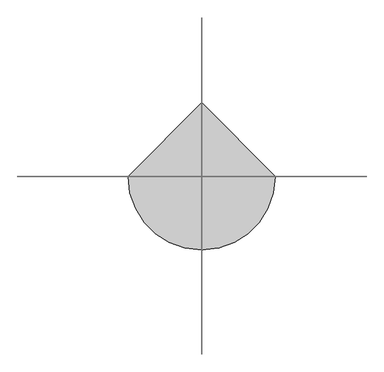
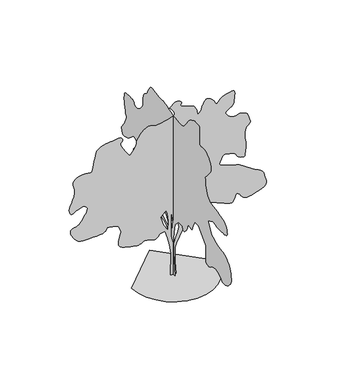
"""IFC4 building model written with IfcOpenShell, lengths in millimetres: geographic element geometry, RPC 木 - 落葉樹 : ブルーベリー エルダー - 4.5 メートル."""

from ifc_helpers import new_model, si_unit, origin, place, context, project, spatial, triangles, source, transform, mapped, element, save


def geographic_element_08da9c25(model_context):
    return source(origin(), model_context, "Body", "Tessellation", [
        triangles([(-0.0014684, 58.7037978, 0.0041346), (-0.0014684, -62.498052, 0.0041346), (-0.0014684, -15.3641626, 565.6129683), (-0.0014684, -1.8971866, 909.0182064), (-0.0014684, -22.0974929, 1104.2884094), (-0.0014684, -75.9650625, 1326.4911255), (-0.0014684, -224.1009287, 1474.6287403), (-0.0014684, -378.970291, 1474.6287403), (-0.0014684, -412.6378218, 1380.3586224), (-0.0014684, -479.9703761, 1387.0936764), (-0.0014684, -554.0404552, 1474.6287403), (-0.0014684, -601.1729708, 1568.8962421), (-0.0014684, -628.1080273, 1663.1638893), (-0.0014684, -702.1755266, 1636.2313763), (-0.0014684, -782.9756092, 1629.4963223), (-0.0014684, -857.0431812, 1797.8338669), (-0.0014684, -910.9107508, 1898.833952), (-0.0014684, -1059.0483656, 1892.1015141), (-0.0014684, -1173.5159426, 1797.8338669), (-0.0014684, -1382.2535648, 1575.6288254), (-0.0014684, -1388.9861481, 1353.4261093), (-0.0014684, -1386.9236286, 1327.021035), (-0.0014684, -1382.3910564, 1295.553479), (-0.0014684, -1377.8561588, 1261.3760593), (-0.0014684, -1375.7936394, 1226.8434288), (-0.0014684, -1378.6786377, 1194.3159811), (-0.0014684, -1388.9861481, 1166.1458982), (-0.0014684, -1409.1860779, 1144.6884144), (-0.0014684, -1434.4711624, 1129.1809307), (-0.0014684, -1458.931152, 1117.9109064), (-0.0014684, -1483.3911415, 1111.8258854), (-0.0014684, -1508.676226, 1111.8658539), (-0.0014684, -1535.6112099, 1118.9734142), (-0.0014684, -1565.0162464, 1134.0884073), (-0.0014684, -1597.723843, 1158.1559063), (-0.0014684, -1638.2812511, 1183.6959171), (-0.0014684, -1688.0263252, 1202.5209309), (-0.0014684, -1742.9539318, 1214.5159836), (-0.0014684, -1799.0589375, 1219.5610245), (-0.0014684, -1852.3364994, 1217.5409443), (-0.0014684, -1898.783955, 1208.3334394), (-0.0014684, -1934.3939907, 1191.8234734), (-0.0014684, -1963.8416119, 1167.0484594), (-0.0014684, -1995.1715309, 1136.2684341), (-0.0014684, -2029.446619, 1104.1908863), (-0.0014684, -2067.729166, 1075.5283916), (-0.0014684, -2111.0741947, 1054.9958513), (-0.0014684, -2160.5442856, 1047.2983561), (-0.0014684, -2217.1992577, 1057.1533504), (-0.0014684, -2275.1493542, 1083.4008762), (-0.0014684, -2327.094294, 1119.5408941), (-0.0014684, -2371.9694618, 1162.2784018), (-0.0014684, -2408.7193989, 1208.3134552), (-0.0014684, -2436.2819607, 1254.348436), (-0.0014684, -2453.5944214, 1297.0834728), (-0.0014684, -2459.6019035, 1333.2260342), (-0.0014684, -2455.754464, 1372.7236233), (-0.0014684, -2445.3120781, 1424.1161259), (-0.0014684, -2429.919413, 1481.9887562), (-0.0014684, -2411.2318909, 1540.9212055), (-0.0014684, -2390.8944695, 1595.4962173), (-0.0014684, -2370.5569027, 1640.2937737), (-0.0014684, -2351.8669098, 1669.8963272), (-0.0014684, -2330.1568977, 1694.4363991), (-0.0014684, -2300.1992786, 1725.2163517), (-0.0014684, -2262.8217636, 1758.5913494), (-0.0014684, -2218.8493023, 1790.903912), (-0.0014684, -2169.1042282, 1818.5039715), (-0.0014684, -2114.4116364, 1837.74146), (-0.0014684, -2055.5966217, 1844.9664551), (-0.0014684, -1994.4066067, 1849.8740044), (-0.0014684, -1932.1564819, 1863.6164795), (-0.0014684, -1869.0239983, 1884.7189705), (-0.0014684, -1805.1839996, 1911.7115089), (-0.0014684, -1740.8139462, 1943.1215103), (-0.0014684, -1676.0888271, 1977.4765354), (-0.0014684, -1611.1887188, 2013.3016743), (-0.0014684, -1469.786158, 2275.9068661), (-0.0014684, -1685.2562908, 2376.9094219), (-0.0014684, -1714.2713802, 2368.3093655), (-0.0014684, -1744.228854, 2360.0643745), (-0.0014684, -1776.0713871, 2352.5268986), (-0.0014684, -1810.7388931, 2346.049387), (-0.0014684, -1849.1765179, 2340.9844345), (-0.0014684, -1892.3265003, 2337.686816), (-0.0014684, -1941.1290447, 2336.5068008), (-0.0014684, -1996.881601, 2336.291843), (-0.0014684, -2057.3441895, 2336.4293346), (-0.0014684, -2118.1616982, 2338.0968201), (-0.0014684, -2174.9742188, 2342.4769306), (-0.0014684, -2223.421843, 2350.7393623), (-0.0014684, -2259.1517841, 2364.0693626), (-0.0014684, -2277.7993378, 2383.6418598), (-0.0014684, -2281.3742649, 2414.4819832), (-0.0014684, -2275.8767807, 2457.2194908), (-0.0014684, -2262.9592552, 2506.4269524), (-0.0014684, -2244.2692623, 2556.7020813), (-0.0014684, -2221.4593174, 2602.6271851), (-0.0014684, -2196.1742329, 2638.7770134), (-0.0014684, -2170.0641987, 2659.7021896), (-0.0014684, -2143.7191498, 2670.2021301), (-0.0014684, -2115.1367374, 2679.2771576), (-0.0014684, -2082.0791622, 2687.9772079), (-0.0014684, -2042.3065899, 2697.4022141), (-0.0014684, -1993.581657, 2708.6021118), (-0.0014684, -1933.6665642, 2722.6021294), (-0.0014684, -1860.3264187, 2740.5021996), (-0.0014684, -1781.7239491, 2758.3022758), (-0.0014684, -1708.0688519, 2773.1522415), (-0.0014684, -1640.1837513, 2787.8522163), (-0.0014684, -1578.8962132, 2805.302314), (-0.0014684, -1525.0287163, 2828.2773651), (-0.0014684, -1479.4062103, 2859.6021973), (-0.0014684, -1442.8536449, 2902.1272179), (-0.0014684, -1414.8411106, 2953.5272781), (-0.0014684, -1393.5411026, 3009.1773697), (-0.0014684, -1377.8361019, 3068.3775352), (-0.0014684, -1366.6061188, 3130.3775299), (-0.0014684, -1358.7336342, 3194.527684), (-0.0014684, -1353.1011292, 3260.0777527), (-0.0014684, -1348.5861431, 3326.3277786), (-0.0014684, -1398.7811897, 3378.2528069), (-0.0014684, -1447.1536732, 3430.0528427), (-0.0014684, -1491.8711472, 3481.6278923), (-0.0014684, -1531.1136646, 3532.8529633), (-0.0014684, -1563.0537209, 3583.577774), (-0.0014684, -1585.8662819, 3633.7529091), (-0.0014684, -1597.723843, 3683.2030884), (-0.0014684, -1593.7187096, 3737.8779488), (-0.0014684, -1572.2812099, 3799.8529449), (-0.0014684, -1536.5912373, 3863.2281464), (-0.0014684, -1489.8311554, 3922.153038), (-0.0014684, -1435.1786774, 3970.7032722), (-0.0014684, -1375.8135509, 4002.9783371), (-0.0014684, -1314.918576, 4013.128299), (-0.0014684, -1258.4585049, 4010.1031929), (-0.0014684, -1210.3634754, 4007.7533363), (-0.0014684, -1170.7484516, 4007.6533424), (-0.0014684, -1139.7309408, 4011.3281181), (-0.0014684, -1117.4309212, 4020.3031517), (-0.0014684, -1103.9633566, 4036.1033501), (-0.0014684, -1099.4483706, 4060.2783279), (-0.0014684, -1101.1558971, 4105.3531929), (-0.0014684, -1104.8659178, 4175.1532928), (-0.0014684, -1108.4583584, 4258.1534592), (-0.0014684, -1109.8133629, 4342.8035248), (-0.0014684, -1106.8083864, 4417.5536133), (-0.0014684, -1097.3283691, 4470.8785561), (-0.0014684, -1079.2483681, 4491.2034782), (-0.0014684, -1052.7858118, 4492.578685), (-0.0014684, -1020.9033102, 4495.6035004), (-0.0014684, -985.6082989, 4498.6286064), (-0.0014684, -948.8982576, 4500.0035225), (-0.0014684, -912.7757532, 4498.07864), (-0.0014684, -879.2456778, 4491.2034782), (-0.0014684, -850.3106707, 4477.7537178), (-0.0014684, -822.8281912, 4461.7535316), (-0.0014684, -792.8706448, 4447.2035477), (-0.0014684, -761.2631264, 4432.1535942), (-0.0014684, -728.8330564, 4414.7534935), (-0.0014684, -696.4030592, 4393.1286507), (-0.0014684, -664.7980116, 4365.3786003), (-0.0014684, -634.8405378, 4329.6034584), (-0.0014684, -604.8054889, 4286.4284775), (-0.0014684, -572.6504748, 4239.8534134), (-0.0014684, -538.7279451, 4193.0283646), (-0.0014684, -503.3903855, 4149.1534264), (-0.0014684, -466.9953687, 4111.403405), (-0.0014684, -429.8928369, 4082.9533974), (-0.0014684, -392.4378193, 4067.0032082), (-0.0014684, -354.0977903, 4061.0282822), (-0.0014684, -314.1102602, 4059.6533661), (-0.0014684, -272.4727218, 4061.703241), (-0.0014684, -229.185175, 4065.9782707), (-0.0014684, -184.2498909, 4071.3282349), (-0.0014684, -137.6653616, 4076.5532066), (-0.0014684, -89.4320684, 4080.4782578), (-0.0014684, -32.5020268, 4087.803392), (-0.0014684, 35.3820291, 4102.1033913), (-0.0014684, 107.0353362, 4120.403437), (-0.0014684, 175.2726409, 4139.7534187), (-0.0014684, 232.909439, 4157.2282242), (-0.0014684, 272.7602224, 4169.8783241), (-0.0014684, 287.6402371, 4174.7283188), (-0.0014684, 295.8277279, 4177.2784538), (-0.0014684, 318.5002539, 4183.6033585), (-0.0014684, 352.8352947, 4191.7034454), (-0.0014684, 396.002827, 4199.553257), (-0.0014684, 445.1803485, 4205.1534966), (-0.0014684, 497.5354013, 4206.5284126), (-0.0014684, 550.2454471, 4201.678418), (-0.0014684, 608.3329988, 4200.728476), (-0.0014684, 675.2555128, 4211.4534027), (-0.0014684, 745.8280947, 4228.1782539), (-0.0014684, 814.8706827, 4245.2533745), (-0.0014684, 877.2006718, 4257.0285278), (-0.0014684, 927.6307331, 4257.8534775), (-0.0014684, 960.9857466, 4242.0782776), (-0.0014684, 983.9932812, 4214.9534798), (-0.0014684, 1006.5283155, 4185.8032242), (-0.0014684, 1028.123291, 4155.1533508), (-0.0014684, 1048.3033092, 4123.4282524), (-0.0014684, 1066.5983408, 4091.1031906), (-0.0014684, 1082.5408997, 4058.6781349), (-0.0014684, 1095.6533987, 4026.6033485), (-0.0014684, 1111.3183582, 3999.2282753), (-0.0014684, 1133.5808802, 3978.353096), (-0.0014684, 1159.9634268, 3960.5283119), (-0.0014684, 1187.9984161, 3942.3532585), (-0.0014684, 1215.2059851, 3920.4031448), (-0.0014684, 1239.1159355, 3891.2531799), (-0.0014684, 1257.255962, 3851.5279884), (-0.0014684, 1268.2685165, 3817.1530518), (-0.0014684, 1273.6285091, 3800.8031776), (-0.0014684, 1275.1009483, 3794.1030052), (-0.0014684, 1274.4534588, 3788.7030441), (-0.0014684, 1273.451049, 3776.252932), (-0.0014684, 1273.8635239, 3748.3528908), (-0.0014684, 1277.4560371, 3696.6528488), (-0.0014684, 1283.7985279, 3637.6029648), (-0.0014684, 1291.9060272, 3591.1778915), (-0.0014684, 1302.7210648, 3554.2528198), (-0.0014684, 1317.1884956, 3523.8279327), (-0.0014684, 1336.2511402, 3496.8278366), (-0.0014684, 1360.8486214, 3470.1527206), (-0.0014684, 1391.9260849, 3440.8027679), (-0.0014684, 1427.2211689, 3411.5778076), (-0.0014684, 1463.2262386, 3387.677813), (-0.0014684, 1498.9912067, 3369.4027657), (-0.0014684, 1533.5812466, 3357.1526413), (-0.0014684, 1566.0512123, 3351.2777092), (-0.0014684, 1595.4587196, 3352.1026588), (-0.0014684, 1620.8612389, 3360.002758), (-0.0014684, 1639.7087803, 3375.502684), (-0.0014684, 1652.8988182, 3396.6528465), (-0.0014684, 1664.6787678, 3420.0528717), (-0.0014684, 1679.2838356, 3442.2776779), (-0.0014684, 1700.9563499, 3459.9027649), (-0.0014684, 1733.936459, 3469.5277588), (-0.0014684, 1782.4638748, 3467.7278687), (-0.0014684, 1840.5514629, 3464.2277916), (-0.0014684, 1897.5815575, 3466.9779144), (-0.0014684, 1950.8390625, 3469.852739), (-0.0014684, 1997.6215267, 3466.7026405), (-0.0014684, 2035.2141449, 3451.4277008), (-0.0014684, 2060.9117043, 3417.9027122), (-0.0014684, 2072.001725, 3360.002758), (-0.0014684, 2074.396637, 3302.252504), (-0.0014684, 2075.4967152, 3266.6526421), (-0.0014684, 2074.8291687, 3243.2026199), (-0.0014684, 2071.9241135, 3221.8774681), (-0.0014684, 2066.3091946, 3192.6275093), (-0.0014684, 2057.5140919, 3145.5024788), (-0.0014684, 2045.0690666, 3070.4524086), (-0.0014684, 2028.7941879, 2993.7774376), (-0.0014684, 2011.3440903, 2941.8274109), (-0.0014684, 1996.4816254, 2904.7273499), (-0.0014684, 1987.9815628, 2872.5772774), (-0.0014684, 1989.6115505, 2835.4772163), (-0.0014684, 2005.1390911, 2783.5271896), (-0.0014684, 2038.3341579, 2706.8522186), (-0.0014684, 2081.1516026, 2626.4521843), (-0.0014684, 2121.1391327, 2566.6770538), (-0.0014684, 2155.4742462, 2522.5771294), (-0.0014684, 2181.326738, 2489.1794586), (-0.0014684, 2195.8742512, 2461.5570168), (-0.0014684, 2196.286726, 2434.7619953), (-0.0014684, 2179.7367187, 2403.841935), (-0.0014684, 2160.4392048, 2371.8244125), (-0.0014684, 2149.859182, 2345.5768867), (-0.0014684, 2141.0441677, 2325.9269234), (-0.0014684, 2127.0467663, 2313.6968559), (-0.0014684, 2100.919146, 2309.7117794), (-0.0014684, 2055.7091148, 2314.7967888), (-0.0014684, 1984.4665157, 2329.7743629), (-0.0014684, 1906.7289642, 2358.6118469), (-0.0014684, 1844.06651, 2399.6994553), (-0.0014684, 1792.5939251, 2445.4995667), (-0.0014684, 1748.4239468, 2488.4719437), (-0.0014684, 1707.671347, 2521.0769302), (-0.0014684, 1666.4437763, 2535.7769051), (-0.0014684, 1620.8612389, 2525.0519783), (-0.0014684, 1576.9086891, 2499.6619583), (-0.0014684, 1542.1411892, 2475.3396057), (-0.0014684, 1515.031216, 2451.8994667), (-0.0014684, 1494.0461597, 2429.166988), (-0.0014684, 1477.653701, 2406.9644188), (-0.0014684, 1464.3237007, 2385.1144444), (-0.0014684, 1452.526165, 2363.44193), (-0.0014684, 1471.2737125, 2344.7718487), (-0.0014684, 1489.9612347, 2326.634293), (-0.0014684, 1508.5336475, 2309.5543762), (-0.0014684, 1526.9262749, 2294.0668041), (-0.0014684, 1545.0862129, 2280.6968353), (-0.0014684, 1562.9512562, 2269.9793209), (-0.0014684, 1580.4612339, 2262.4393742), (-0.0014684, 1599.1313152, 2259.024321), (-0.0014684, 1619.331245, 2258.1993713), (-0.0014684, 1639.2963055, 2256.7868122), (-0.0014684, 1657.2588718, 2251.6042797), (-0.0014684, 1671.4513195, 2239.4717354), (-0.0014684, 1680.1087852, 2217.2092861), (-0.0014684, 1681.4637897, 2181.6392189), (-0.0014684, 1676.9863014, 2141.9842266), (-0.0014684, 1669.5664055, 2107.6292015), (-0.0014684, 1659.5537899, 2075.6315907), (-0.0014684, 1647.3038109, 2043.0441902), (-0.0014684, 1633.1712433, 2006.9215405), (-0.0014684, 1617.5037403, 1964.3241405), (-0.0014684, 1600.6613091, 1912.3015892), (-0.0014684, 1583.268766, 1853.7415009), (-0.0014684, 1567.0537674, 1795.0639778), (-0.0014684, 1554.0188072, 1738.6264343), (-0.0014684, 1546.1662342, 1686.7788723), (-0.0014684, 1545.4986877, 1641.8837929), (-0.0014684, 1554.0188072, 1606.2938141), (-0.0014684, 1573.728796, 1582.3637341), (-0.0014684, 1599.1112583, 1566.4212479), (-0.0014684, 1623.4337563, 1552.9562267), (-0.0014684, 1646.8737499, 1541.5487835), (-0.0014684, 1669.606374, 1531.7937103), (-0.0014684, 1691.8087978, 1523.2737362), (-0.0014684, 1713.6589176, 1515.5787117), (-0.0014684, 1735.331432, 1508.2936913), (-0.0014684, 1758.2389, 1518.0512352), (-0.0014684, 1780.0888744, 1525.7462597), (-0.0014684, 1799.8189201, 1529.318716), (-0.0014684, 1816.3664566, 1526.7087009), (-0.0014684, 1828.676461, 1515.8536949), (-0.0014684, 1835.6840275, 1494.6911785), (-0.0014684, 1836.331517, 1461.1611031), (-0.0014684, 1830.501495, 1425.4711304), (-0.0014684, 1819.3715057, 1398.2636341), (-0.0014684, 1803.8239082, 1378.1211136), (-0.0014684, 1784.7414974, 1363.6336258), (-0.0014684, 1763.0089577, 1353.3861408), (-0.0014684, 1739.5114094, 1345.9660995), (-0.0014684, 1715.128886, 1339.9586174), (-0.0014684, 1703.5663651, 1332.6360992), (-0.0014684, 1691.8864094, 1324.6660915), (-0.0014684, 1679.9712936, 1315.4011047), (-0.0014684, 1667.701403, 1304.1910332), (-0.0014684, 1654.9613377, 1290.3910034), (-0.0014684, 1641.6313374, 1273.3510551), (-0.0014684, 1627.5962929, 1252.4235535), (-0.0014684, 1608.2588104, 1230.1234612), (-0.0014684, 1580.0887276, 1209.2360006), (-0.0014684, 1544.5563034, 1189.5259392), (-0.0014684, 1503.1336864, 1170.7584074), (-0.0014684, 1457.2962227, 1152.6983906), (-0.0014684, 1408.5135899, 1135.1084032), (-0.0014684, 1358.2585178, 1117.7559013), (-0.0014684, 1196.6559546, 1212.0234758), (-0.0014684, 1035.0533186, 1090.8208448), (-0.0014684, 1013.4382862, 1088.0133854), (-0.0014684, 992.0007866, 1085.6783535), (-0.0014684, 970.9182798, 1084.2833805), (-0.0014684, 950.3632845, 1084.3033648), (-0.0014684, 930.5182749, 1086.2083357), (-0.0014684, 911.5532261, 1090.4683954), (-0.0014684, 893.6506851, 1097.5558989), (-0.0014684, 877.0431959, 1106.938393), (-0.0014684, 861.3756929, 1117.3809242), (-0.0014684, 845.9456755, 1128.295883), (-0.0014684, 830.0456285, 1139.0934071), (-0.0014684, 812.9656391, 1149.1834162), (-0.0014684, 794.0031338, 1157.9784462), (-0.0014684, 772.4481268, 1164.8884169), (-0.0014684, 748.1855816, 1170.2684664), (-0.0014684, 721.8005642, 1174.9409283), (-0.0014684, 693.6505383, 1179.0234552), (-0.0014684, 664.0855551, 1182.6359528), (-0.0014684, 633.4605349, 1185.8934574), (-0.0014684, 602.1304705, 1188.9184181), (-0.0014684, 570.4454495, 1191.8234734), (-0.0014684, 361.7077909, 1131.2209225), (-0.0014684, 186.6391528, 1003.2857809), (-0.0014684, 92.3710696, 848.418199), (-0.0014684, 45.2367873, 552.1454401), (-0.0013758, 65.4370532, 1097.5558989), (-0.0013758, 166.4388778, 1313.0261044), (-0.0013758, 4.8361539, 1380.3586224), (-0.0013882, 307.8402577, 1171.6234709), (-0.0013882, 469.4428937, 1279.3585373), (-0.0013882, 597.3779626, 1286.0909752), (-0.0013882, 705.1130653, 1346.6910553), (-0.0013882, 699.3030275, 1349.8135391), (-0.0013882, 693.2555769, 1354.3485821), (-0.0013882, 686.7405676, 1361.7110687), (-0.0013882, 679.5155725, 1373.3110874), (-0.0013882, 671.3480478, 1390.5686096), (-0.0013882, 662.0055222, 1414.8911076), (-0.0013882, 651.2454958, 1447.6936111), (-0.0013882, 642.6479828, 1480.1036968), (-0.0013882, 639.3505096, 1503.3287327), (-0.0013882, 640.4680286, 1518.8962418), (-0.0013882, 645.1205063, 1528.3386887), (-0.0013882, 652.425511, 1533.1862125), (-0.0013882, 661.4930534, 1534.9737488), (-0.0013882, 671.4480417, 1535.2286751), (-0.0013882, 678.1805523, 1616.0288303), (-0.0013882, 597.3779626, 1669.8963272), (-0.0013882, 422.3103418, 1521.7611832), (-0.0013882, 301.1077472, 1380.3586224), (-0.0013882, 220.3061749, 1265.8910454), (-0.0013882, 139.504866, 1084.0883343), (66.6360534, 0.0002629, 0.0), (-68.0330566, 0.0002629, 0.0), (-61.2998012, 0.0002272, 552.142933), (-94.9670776, 0.0002139, 794.5456152), (-142.1008648, 0.0002005, 996.5483288), (-202.7016535, 0.0001916, 1178.3509672), (-323.9027584, 0.0001916, 1164.8859461), (-344.1627863, 0.0001916, 1136.3209019), (-364.7752999, 0.000196, 1109.5258804), (-386.0952922, 0.000196, 1086.2633469), (-408.4753215, 0.000196, 1068.3008532), (-432.2678372, 0.0002005, 1057.4058786), (-457.8253615, 0.0002005, 1055.3433592), (-485.5053944, 0.000196, 1063.8833176), (-514.9529065, 0.000196, 1076.7408903), (-545.4604194, 0.000196, 1086.7733448), (-576.8504728, 0.000196, 1094.448385), (-608.9454978, 0.000196, 1100.2409094), (-641.5730484, 0.000196, 1104.6184038), (-674.5530121, 0.000196, 1108.0533686), (-707.7105812, 0.000196, 1111.0183765), (-735.2131176, 0.000196, 1095.3133759), (-763.2456362, 0.000196, 1080.6083868), (-792.3406626, 0.000196, 1067.9083626), (-823.0231647, 0.000196, 1058.210844), (-855.8256683, 0.0002005, 1052.5183136), (-891.280699, 0.0002005, 1051.8308556), (-929.9132246, 0.0002005, 1057.1508797), (-979.8558157, 0.000196, 1066.7883728), (-1044.1658438, 0.000196, 1079.0183676), (-1115.7808765, 0.000196, 1094.7833937), (-1187.630924, 0.000196, 1115.0233646), (-1252.6485397, 0.0001916, 1140.6808828), (-1303.7660591, 0.0001916, 1172.6984053), (-1333.9185791, 0.0001871, 1212.0184616), (-1343.6560661, 0.0001871, 1258.8785374), (-1340.9085594, 0.0001827, 1310.6835148), (-1329.6785763, 0.0001782, 1364.141153), (-1313.9735756, 0.0001782, 1415.9461304), (-1297.7985455, 0.0001738, 1462.8062061), (-1285.1560032, 0.0001738, 1501.4186749), (-1280.0510822, 0.0001693, 1528.4911503), (-1282.3885849, 0.0001693, 1551.6362492), (-1288.8460396, 0.0001693, 1579.2562202), (-1298.6035835, 0.0001648, 1609.2337509), (-1310.8335056, 0.0001648, 1639.4462963), (-1324.7136177, 0.0001604, 1667.7737823), (-1339.4160633, 0.0001604, 1692.0964256), (-1354.121125, 0.0001604, 1710.2938614), (-1373.4561367, 0.0001604, 1723.3488785), (-1401.6286903, 0.0001559, 1733.9289013), (-1437.1586437, 0.0001559, 1742.4488754), (-1478.5811153, 0.0001559, 1749.3189503), (-1524.4187244, 0.0001559, 1754.9539261), (-1573.2012119, 0.0001559, 1759.7639523), (-1623.456284, 0.0001559, 1764.1613583), (-1631.2713593, 0.0001559, 1738.3664211), (-1642.6763317, 0.0001604, 1713.631303), (-1661.2663307, 0.0001604, 1691.0164043), (-1690.6363403, 0.0001604, 1671.5813988), (-1734.3739323, 0.0001604, 1656.386396), (-1796.0739452, 0.0001648, 1646.4938313), (-1879.3290379, 0.0001648, 1642.9588726), (-1971.5741341, 0.0001648, 1640.6613384), (-2057.4616241, 0.0001648, 1636.1262955), (-2136.396777, 0.0001648, 1632.8888477), (-2207.7943085, 0.0001648, 1634.478867), (-2271.0667545, 0.0001648, 1644.4313118), (-2325.619384, 0.0001604, 1666.2812862), (-2370.8693836, 0.0001604, 1703.5614235), (-2411.8019142, 0.0001559, 1752.5588688), (-2450.9643494, 0.0001559, 1805.3264328), (-2484.1219185, 0.0001515, 1859.0389973), (-2507.0269157, 0.000147, 1910.8640316), (-2515.4519829, 0.0001426, 1957.9790337), (-2505.1520302, 0.0001426, 1997.554089), (-2471.8720848, 0.0001426, 2026.7640793), (-2428.4668854, 0.0001381, 2045.1190636), (-2390.1269291, 0.0001381, 2056.5266521), (-2356.1468811, 0.0001381, 2064.7515862), (-2325.816901, 0.0001381, 2073.5666004), (-2298.4317993, 0.0001381, 2086.7391975), (-2273.2843517, 0.0001337, 2108.0367348), (-2249.6667526, 0.0001337, 2141.2342724), (-2221.7142437, 0.0001292, 2184.9518074), (-2187.6342018, 0.0001292, 2233.7342949), (-2152.8467903, 0.0001247, 2285.2267914), (-2122.7717365, 0.0001203, 2337.0718826), (-2102.826733, 0.0001203, 2386.9169506), (-2098.4291817, 0.0001158, 2432.401965), (-2114.9992458, 0.0001158, 2471.1718369), (-2145.426749, 0.0001114, 2498.537027), (-2178.6816959, 0.0001114, 2512.8271431), (-2214.2917316, 0.0001114, 2516.2269356), (-2251.7868267, 0.0001114, 2510.9019699), (-2290.6968063, 0.0001114, 2499.0494957), (-2330.5468449, 0.0001114, 2482.831881), (-2370.8693836, 0.0001158, 2464.439399), (-2399.569376, 0.0001158, 2448.8118645), (-2427.3294548, 0.0001158, 2434.6593853), (-2453.2020035, 0.0001158, 2423.4494591), (-2476.2471085, 0.0001158, 2416.6569958), (-2495.5270363, 0.0001158, 2415.7544346), (-2510.1020187, 0.0001158, 2422.2118893), (-2519.0020569, 0.0001158, 2437.5044151), (-2525.7269371, 0.0001158, 2456.4494797), (-2533.1520653, 0.0001158, 2474.4518692), (-2539.5019684, 0.0001114, 2493.8669632), (-2543.0270439, 0.0001114, 2517.0518852), (-2541.977108, 0.0001114, 2546.3521317), (-2534.5519798, 0.0001069, 2584.15215), (-2519.0020569, 0.0001025, 2632.7770889), (-2498.1969315, 0.0001025, 2684.6521202), (-2477.0345604, 9.8e-05, 2732.0771324), (-2456.8145737, 9.8e-05, 2777.1272896), (-2438.8319504, 9.36e-05, 2821.9271713), (-2424.3844311, 8.91e-05, 2868.6522263), (-2414.7643787, 8.91e-05, 2919.3523293), (-2411.2693886, 8.47e-05, 2976.1773491), (-2415.2169674, 8.02e-05, 3030.6775108), (-2424.696912, 8.02e-05, 3074.9274261), (-2436.1819668, 7.57e-05, 3111.8774963), (-2446.1344116, 7.57e-05, 3144.4525429), (-2451.0245201, 7.13e-05, 3175.6276749), (-2447.311956, 7.13e-05, 3208.3274231), (-2431.4719345, 6.68e-05, 3245.527478), (-2401.6519524, 6.68e-05, 3281.1526291), (-2361.1144558, 6.24e-05, 3307.9527374), (-2313.9793968, 6.24e-05, 3326.977739), (-2264.3718143, 6.24e-05, 3339.2775696), (-2216.4142765, 6.24e-05, 3345.9277451), (-2174.2267353, 6.24e-05, 3348.0026184), (-2141.9342297, 6.24e-05, 3346.5277084), (-2114.2341763, 6.24e-05, 3341.002755), (-2084.4141941, 6.24e-05, 3332.902668), (-2054.4766319, 6.24e-05, 3326.2027863), (-2026.4241291, 6.24e-05, 3324.9275734), (-2002.2565636, 6.24e-05, 3333.0776573), (-1983.9815163, 6.24e-05, 3354.6527939), (-1973.5965397, 5.79e-05, 3393.652739), (-1964.8216393, 5.35e-05, 3450.0277863), (-1951.2165104, 5.35e-05, 3517.3777451), (-1934.5515392, 4.9e-05, 3590.1279556), (-1916.5889729, 4.46e-05, 3662.7528831), (-1899.0965813, 4.01e-05, 3729.7278648), (-1883.8440239, 3.56e-05, 3785.5279472), (-1872.5939838, 3.12e-05, 3824.6031784), (-1852.5114887, 3.12e-05, 3852.8781967), (-1813.3489082, 3.12e-05, 3879.4030312), (-1760.7564789, 2.67e-05, 3903.2280304), (-1700.3914135, 2.67e-05, 3923.3782539), (-1637.906274, 2.67e-05, 3938.9531754), (-1578.9537678, 2.67e-05, 3948.9781448), (-1529.1887821, 2.67e-05, 3952.5282188), (-1482.7811497, 2.67e-05, 3955.978299), (-1432.4861092, 2.67e-05, 3963.6781197), (-1381.8386192, 2.67e-05, 3971.6032173), (-1334.3710224, 2.23e-05, 3975.7782532), (-1293.6160973, 2.67e-05, 3972.1531837), (-1263.1109825, 2.67e-05, 3956.7782501), (-1246.3835152, 2.67e-05, 3925.6031181), (-1245.9735111, 3.12e-05, 3891.2531799), (-1257.1035004, 3.12e-05, 3865.2780212), (-1272.3560577, 3.12e-05, 3842.0279869), (-1284.3134674, 3.56e-05, 3815.8281326), (-1285.5485664, 3.56e-05, 3781.0029327), (-1268.6459644, 4.01e-05, 3731.9530197), (-1226.1859108, 4.46e-05, 3663.0028679), (-1175.7534513, 4.9e-05, 3589.303006), (-1137.6884056, 4.9e-05, 3530.2028343), (-1108.6933731, 5.35e-05, 3486.3028976), (-1085.4708807, 5.35e-05, 3458.2028687), (-1064.7208391, 5.79e-05, 3446.4527138), (-1043.1458479, 5.35e-05, 3451.6776855), (-1017.4482885, 5.35e-05, 3474.4527489), (-990.2407923, 5.35e-05, 3507.3527756), (-966.3282984, 4.9e-05, 3542.2529709), (-945.7157484, 4.9e-05, 3578.7027809), (-928.403215, 4.46e-05, 3616.2028175), (-914.3857567, 4.46e-05, 3654.2778191), (-903.6682423, 4.01e-05, 3692.477813), (-896.2457302, 4.01e-05, 3730.3281189), (-882.6607309, 3.56e-05, 3773.9530724), (-855.1781788, 3.12e-05, 3826.1530838), (-816.3881773, 3.12e-05, 3881.5531906), (-768.880612, 2.67e-05, 3934.7281425), (-715.2480572, 2.23e-05, 3980.2282722), (-658.0830145, 2.23e-05, 4012.6533279), (-599.9754785, 2.23e-05, 4026.6033485), (-552.8204352, 2.23e-05, 4024.7781693), (-521.215424, 2.23e-05, 4016.1031174), (-496.7928958, 2.23e-05, 4004.503244), (-471.1953667, 2.23e-05, 3993.8533127), (-436.0553604, 2.23e-05, 3988.0280869), (-383.0128132, 2.23e-05, 3990.9032021), (-303.7027378, 2.23e-05, 4006.4031281), (-214.7551692, 2.23e-05, 4026.5783501), (-138.763614, 2.23e-05, 4042.5282486), (-76.3173075, 1.78e-05, 4056.5782631), (-28.0055217, 1.78e-05, 4071.1032486), (5.5830293, 1.78e-05, 4088.4533524), (23.8594698, 1.78e-05, 4110.9784309), (26.2347699, 1.34e-05, 4141.0533394), (18.3040142, 1.34e-05, 4173.7283798), (6.4862053, 8.9e-06, 4202.8533463), (-8.5707069, 8.9e-06, 4229.0534912), (-26.219021, 8.9e-06, 4252.8784904), (-45.810535, 4.5e-06, 4274.9533058), (-66.6978047, 4.5e-06, 4295.8284851), (-88.2330682, 4.5e-06, 4316.1284088), (-60.8870493, 4.5e-06, 4341.9035797), (-33.9532782, 0.0, 4366.5035316), (-7.8441564, 0.0, 4388.753627), (17.0283131, 0.0, 4407.4536484), (40.2517809, 0.0, 4421.4536659), (61.4140475, -4.5e-06, 4429.5534622), (80.1028141, -4.5e-06, 4430.6036888), (99.5373291, -4.5e-06, 4426.853627), (121.7990971, 0.0, 4421.2286797), (144.7671174, 0.0, 4413.4535728), (166.3221335, 0.0, 4403.3536079), (184.343399, 0.0, 4390.653511), (196.7109036, 0.0, 4375.1285866), (201.3046639, 0.0, 4356.5285591), (197.1231604, 4.5e-06, 4339.6534264), (187.641399, 4.5e-06, 4327.8285667), (177.4531401, 4.5e-06, 4318.7285408), (171.1516352, 4.5e-06, 4309.9784935), (173.3306447, 4.5e-06, 4299.2035698), (188.5838924, 4.5e-06, 4284.1033287), (221.5051751, 8.9e-06, 4262.2784981), (265.7927153, 8.9e-06, 4240.0534012), (311.140238, 8.9e-06, 4223.8285194), (356.135275, 8.9e-06, 4211.3784073), (399.3628326, 8.9e-06, 4200.4784912), (439.4103518, 1.34e-05, 4188.8533287), (474.8628754, 1.34e-05, 4174.2783463), (504.3103875, 1.34e-05, 4154.528389), (527.7304333, 1.34e-05, 4129.0781982), (546.555447, 1.78e-05, 4099.4032654), (561.5529327, 1.78e-05, 4066.203257), (573.4879601, 2.23e-05, 4030.1531319), (583.1279603, 2.23e-05, 3991.9781364), (591.2354596, 2.67e-05, 3952.4032265), (598.577962, 2.67e-05, 3912.1280685), (692.8455729, 2.23e-05, 3999.6532494), (692.2180676, 2.23e-05, 4003.2033234), (691.118062, 2.23e-05, 4013.1033005), (690.7255714, 2.23e-05, 4028.2782463), (692.2180676, 2.23e-05, 4047.7282219), (696.7730221, 1.78e-05, 4070.3282959), (705.5680521, 1.78e-05, 4095.0782387), (719.7805567, 1.78e-05, 4120.8534096), (736.0730942, 1.34e-05, 4147.7032242), (751.1906307, 1.34e-05, 4174.7783157), (766.4231312, 8.9e-06, 4199.8282402), (783.0706615, 8.9e-06, 4220.678421), (802.4256575, 8.9e-06, 4235.0284172), (825.7856415, 8.9e-06, 4240.6533646), (854.4482088, 8.9e-06, 4235.3283989), (884.2282225, 8.9e-06, 4222.4283142), (910.4757483, 8.9e-06, 4207.0283821), (933.7782503, 1.34e-05, 4189.5782845), (954.7232655, 1.34e-05, 4170.4782875), (973.9032721, 1.34e-05, 4150.1283669), (991.9032635, 1.34e-05, 4128.9782043), (1009.3183342, 1.78e-05, 4107.4033585), (1013.7732948, 1.78e-05, 4086.0282097), (1018.9957958, 1.78e-05, 4066.2282555), (1025.7482906, 1.78e-05, 4049.6281059), (1034.7983196, 2.23e-05, 4037.7782478), (1046.910807, 2.23e-05, 4032.3032913), (1062.8508224, 2.23e-05, 4034.7781403), (1083.3858335, 2.23e-05, 4046.8032784), (1105.9033545, 1.78e-05, 4067.7281639), (1128.3008972, 1.78e-05, 4093.828315), (1152.1133972, 1.78e-05, 4122.0533363), (1178.8709209, 1.34e-05, 4149.3534142), (1210.1034622, 1.34e-05, 4172.628447), (1247.3434856, 1.34e-05, 4188.8533287), (1292.120985, 1.34e-05, 4194.9282486), (1340.4335884, 8.9e-06, 4200.0782249), (1385.9186028, 8.9e-06, 4211.3534088), (1426.5736794, 8.9e-06, 4222.5033096), (1460.3986496, 8.9e-06, 4227.2783089), (1485.388694, 8.9e-06, 4219.4784943), (1499.543644, 1.34e-05, 4192.8033783), (1500.85868, 1.34e-05, 4141.0533394), (1496.0287422, 1.78e-05, 4077.628141), (1491.9061741, 2.23e-05, 4020.1781593), (1486.7236416, 2.67e-05, 3968.9780869), (1478.7161362, 2.67e-05, 3924.2532005), (1466.111237, 3.12e-05, 3886.2531944), (1447.1485863, 3.12e-05, 3855.2030548), (1420.05867, 3.12e-05, 3831.3280586), (1386.1536175, 3.56e-05, 3811.7280922), (1350.8386219, 3.56e-05, 3792.5031029), (1318.4660339, 3.56e-05, 3772.3278809), (1293.3985233, 3.56e-05, 3749.9030869), (1279.9910568, 4.01e-05, 3723.9529266), (1282.6010719, 4.01e-05, 3693.1530624), (1305.5884769, 4.46e-05, 3656.2529892), (1339.7660419, 4.46e-05, 3620.9528183), (1372.8836426, 4.9e-05, 3594.8529579), (1404.7061188, 4.9e-05, 3576.4029213), (1434.9961304, 4.9e-05, 3564.0778015), (1463.5211334, 4.9e-05, 3556.3279839), (1490.0411716, 4.9e-05, 3551.6529785), (1514.3261719, 4.9e-05, 3548.5278786), (1534.9186649, 4.9e-05, 3550.0027885), (1552.0962502, 4.9e-05, 3557.8278923), (1568.2112549, 4.9e-05, 3568.4778236), (1585.6263256, 4.9e-05, 3578.4527962), (1606.6888481, 4.9e-05, 3584.152739), (1633.7613235, 4.9e-05, 3582.1028641), (1669.1938992, 4.9e-05, 3568.7278084), (1706.7689312, 4.9e-05, 3552.8279068), (1738.9239452, 4.9e-05, 3542.9279297), (1766.0138615, 4.9e-05, 3535.1528229), (1788.3938908, 4.9e-05, 3525.6028244), (1806.4140118, 5.35e-05, 3510.4278786), (1820.4314701, 5.35e-05, 3485.6776451), (1830.7965351, 5.79e-05, 3447.5276482), (1843.1639488, 5.79e-05, 3405.1526184), (1859.6539307, 6.24e-05, 3369.1527809), (1875.3189629, 6.24e-05, 3337.6276703), (1885.2139984, 6.24e-05, 3308.7026917), (1884.3890488, 6.68e-05, 3280.4526718), (1867.8990669, 6.68e-05, 3251.0527222), (1830.7965351, 7.13e-05, 3218.5776695), (1790.6914249, 7.13e-05, 3174.2274696), (1766.368927, 7.57e-05, 3114.4526299), (1754.6488575, 8.02e-05, 3045.2524933), (1752.3514687, 8.47e-05, 2972.6522736), (1756.2964314, 8.91e-05, 2902.6271873), (1763.3064686, 9.36e-05, 2841.2021576), (1770.196455, 9.36e-05, 2794.3771088), (1774.2014431, 9.8e-05, 2756.2771088), (1775.0263927, 9.8e-05, 2717.1021744), (1773.198888, 0.0001025, 2677.0520027), (1769.2539253, 0.0001025, 2636.3021645), (1763.7189434, 0.0001069, 2595.0270676), (1757.121381, 0.0001069, 2553.3769936), (1749.9963799, 0.0001114, 2511.5769287), (1751.0764011, 0.0001114, 2490.1945129), (1749.9764683, 0.0001158, 2470.407058), (1744.5189526, 0.0001158, 2453.7993507), (1732.5238998, 0.0001158, 2441.9619919), (1711.8138268, 0.0001158, 2436.4844193), (1680.2063084, 0.0001158, 2438.9569427), (1635.5263321, 0.0001158, 2450.971907), (1592.8687614, 0.0001158, 2472.329615), (1564.6988239, 0.0001114, 2499.8145653), (1544.8911667, 0.0001114, 2530.4769379), (1527.3211636, 0.0001069, 2561.3770866), (1505.8637524, 0.0001069, 2589.5771095), (1474.3961964, 0.0001069, 2612.1021881), (1426.7911079, 0.0001069, 2626.0522087), (1373.8061153, 0.0001025, 2635.8521919), (1329.4210339, 0.0001025, 2646.0271523), (1292.338559, 0.0001025, 2653.6019806), (1261.2609501, 0.0001025, 2655.6521461), (1234.8984604, 0.0001025, 2649.2022491), (1211.9484804, 0.0001025, 2631.3521759), (1191.1209726, 0.0001069, 2599.1021095), (1170.9584679, 0.0001069, 2559.6521919), (1152.6834206, 0.0001114, 2522.5521309), (1139.0008982, 0.0001114, 2488.5071159), (1132.6209097, 0.0001158, 2458.2345451), (1136.2509207, 0.0001158, 2432.4394627), (1152.6034109, 0.0001158, 2411.8269127), (1184.3859186, 0.0001203, 2397.1044102), (1219.3110397, 0.0001203, 2386.6219105), (1246.1060612, 0.0001203, 2377.5519699), (1269.016, 0.0001203, 2368.8369495), (1292.2785336, 0.0001203, 2359.4119434), (1320.1359901, 0.0001203, 2348.2243996), (1356.8260471, 0.0001203, 2334.2067959), (1406.5911781, 0.0001247, 2316.3044003), (1459.7311031, 0.0001247, 2299.7343361), (1505.2162628, 0.0001247, 2288.4668552), (1545.2837299, 0.0001247, 2279.5543179), (1582.1713039, 0.0001247, 2270.0518456), (1618.1137321, 0.0001247, 2257.01674), (1655.3537556, 0.0001292, 2237.5042683), (1696.128883, 0.0001292, 2208.5692612), (1938.5315289, 0.0001381, 2040.2315712), (1981.0741356, 0.0001426, 2013.7116783), (2030.6815727, 0.0001426, 1989.6615475), (2082.8791134, 0.0001426, 1964.7890831), (2133.1942108, 0.000147, 1935.7940506), (2177.1467606, 0.000147, 1899.3789768), (2210.2642159, 0.0001515, 1852.246534), (2228.0692337, 0.0001559, 1791.0938713), (2241.2617424, 0.0001604, 1726.50886), (2258.5768192, 0.0001604, 1670.1688396), (2272.5942776, 0.0001648, 1620.4237656), (2275.8917507, 0.0001693, 1575.6237385), (2261.0493427, 0.0001693, 1534.1236553), (2220.6493378, 0.0001738, 1494.2737621), (2147.2692238, 0.0001738, 1454.4237236), (2059.4391197, 0.0001782, 1418.5387047), (1980.5615215, 0.0001782, 1391.6035755), (1910.5189945, 0.0001782, 1373.5036629), (1849.1914879, 0.0001782, 1364.121096), (1796.4614216, 0.0001782, 1363.3361149), (1752.2138317, 0.0001782, 1371.0311394), (1716.3288128, 0.0001782, 1387.0885895), (1685.0163345, 0.0001782, 1414.9836891), (1654.6488567, 0.0001738, 1452.773679), (1625.3388725, 0.0001738, 1492.2137135), (1597.2087582, 0.0001693, 1525.0561855), (1570.3712975, 0.0001693, 1543.0562496), (1544.9487213, 0.0001693, 1537.973711), (1521.0587551, 0.0001738, 1501.5561665), (1500.85868, 0.0001738, 1451.6536892), (1484.7811729, 0.0001782, 1411.5286674), (1470.3512398, 0.0001782, 1381.0610504), (1455.0986824, 0.0001782, 1360.1360195), (1436.5486519, 0.0001827, 1348.6310532), (1412.2236832, 0.0001827, 1346.4335129), (1379.656049, 0.0001827, 1353.4210224), (1340.768597, 0.0001782, 1366.1410309), (1299.4060055, 0.0001782, 1380.9835842), (1255.9810398, 0.0001782, 1397.5911461), (1210.9085003, 0.0001782, 1415.6111217), (1164.5984636, 0.0001738, 1434.6936779), (1117.4658754, 0.0001738, 1454.4811329), (1069.9183416, 0.0001738, 1474.6236534), (746.7130697, 0.0001648, 1609.2913055), (558.1779571, 0.0001693, 1528.4911503), (416.7753236, 0.0001827, 1339.9535305), (241.7051957, 0.000196, 1084.0833927), (73.3693089, 0.0002139, 787.8131046), (46.4355377, 0.0002183, 686.8105488), (46.4355377, 0.0002272, 558.8754436), (46.4355377, 0.000245, 289.537723), (-0.6985081, 8.02e-05, 760.8781208), (66.6360534, 6.68e-05, 949.4157406), (120.5033459, 5.79e-05, 1070.6158281), (140.7033666, 5.35e-05, 1178.3509672), (120.5033459, 4.46e-05, 1299.5535255), (59.9020486, 4.46e-05, 1326.4885094), (49.8315377, 4.46e-05, 1318.123613), (39.937783, 4.46e-05, 1311.5285213), (30.397025, 4.46e-05, 1308.4660629), (21.3865171, 4.46e-05, 1310.7035717), (13.0826351, 4.46e-05, 1320.008527), (5.6620545, 4.46e-05, 1338.1485535), (-0.6985081, 4.01e-05, 1366.8886597), (-6.8627806, 4.01e-05, 1401.5160519), (-13.7337354, 4.01e-05, 1436.1462055), (-21.1935919, 3.56e-05, 1470.7762138), (-29.1245236, 3.56e-05, 1505.4037514), (-37.408779, 3.12e-05, 1540.0337597), (-45.9287872, 3.12e-05, 1574.663768), (-54.5662914, 2.67e-05, 1609.2913055), (-61.2998012, 4.9e-05, 1279.3535957), (-54.5662914, 6.24e-05, 1003.2833101), (-128.634354, 8.47e-05, 1185.0859486), (-121.9003446, 7.13e-05, 1420.7561565), (-142.1008648, 6.24e-05, 1609.2913055), (-175.7681412, 5.35e-05, 1717.0264446), (-243.102694, 5.79e-05, 1649.6913105), (-310.4377373, 6.24e-05, 1575.6237385), (-236.368948, 7.57e-05, 1353.4210224), (-1016.5758127, 0.0, 0.0044197), (-989.7007816, -232.9319304, 0.0044197), (-913.1607588, -446.842856, 0.0044197), (-793.0856026, -635.6029913, 0.0044197), (-635.6029913, -793.0856026, 0.0044197), (-446.842856, -913.1607588, 0.0044197), (-232.9319304, -989.7007816, 0.0044197), (4.44e-05, -1016.5758127, 0.0044197), (232.9319304, -989.7007816, 0.0044197), (446.842856, -913.1607588, 0.0044197), (635.6029913, -793.0856026, 0.0044197), (793.0856026, -635.6029913, 0.0044197), (913.1607588, -446.842856, 0.0044197), (989.7007816, -232.9319304, 0.0044197), (1016.5758127, 8.91e-05, 0.0044197), (-0.0001333, 1016.5758127, 0.0044197)], [[379, 1, 382], [380, 404, 405], [379, 382, 380], [378, 379, 380], [404, 380, 381], [380, 405, 406], [377, 378, 380], [377, 380, 406], [376, 377, 406], [376, 406, 383], [376, 383, 384], [375, 376, 384], [375, 384, 385], [374, 375, 385], [1, 2, 3], [373, 374, 385], [373, 385, 386], [372, 373, 386], [371, 372, 386], [370, 371, 386], [8, 9, 10], [8, 10, 11], [369, 370, 386], [14, 15, 16], [13, 14, 16], [368, 369, 386], [8, 11, 12], [367, 368, 386], [8, 12, 13], [351, 352, 353], [404, 381, 382], [403, 404, 382], [148, 149, 150], [147, 148, 150], [147, 150, 151], [146, 147, 151], [146, 151, 152], [146, 152, 153], [146, 153, 154], [145, 146, 154], [145, 154, 155], [145, 155, 156], [145, 156, 157], [145, 157, 158], [144, 145, 158], [144, 158, 159], [144, 159, 160], [144, 160, 161], [144, 161, 162], [144, 162, 163], [143, 144, 163], [143, 163, 164], [143, 164, 165], [142, 143, 165], [142, 165, 166], [141, 142, 166], [141, 166, 167], [141, 167, 168], [141, 168, 169], [140, 141, 169], [366, 367, 386], [350, 351, 353], [7, 8, 13], [92, 93, 94], [91, 92, 94], [91, 94, 95], [90, 91, 95], [90, 95, 96], [89, 90, 96], [89, 96, 97], [88, 89, 97], [88, 97, 98], [88, 98, 99], [88, 99, 100], [88, 100, 101], [88, 101, 102], [88, 102, 103], [87, 88, 103], [87, 103, 104], [87, 104, 105], [86, 87, 105], [86, 105, 106], [85, 86, 106], [84, 85, 106], [84, 106, 107], [83, 84, 107], [82, 83, 107], [81, 82, 107], [81, 107, 108], [80, 81, 108], [79, 80, 108], [79, 108, 109], [79, 109, 110], [78, 79, 110], [78, 110, 111], [78, 111, 112], [78, 112, 113], [78, 113, 114], [349, 350, 353], [271, 272, 273], [270, 271, 273], [270, 273, 274], [269, 270, 274], [269, 274, 275], [268, 269, 275], [268, 275, 276], [267, 268, 276], [266, 267, 276], [265, 266, 276], [264, 265, 276], [263, 264, 276], [262, 263, 276], [262, 276, 277], [262, 277, 278], [261, 262, 278], [261, 278, 279], [260, 261, 279], [260, 279, 280], [259, 260, 280], [259, 280, 281], [258, 259, 281], [258, 281, 282], [327, 328, 329], [327, 329, 330], [326, 327, 330], [326, 330, 331], [325, 326, 331], [325, 331, 332], [324, 325, 332], [324, 332, 333], [324, 333, 334], [324, 334, 335], [324, 335, 336], [324, 336, 337], [324, 337, 338], [323, 324, 338], [322, 323, 338], [322, 338, 339], [321, 322, 339], [321, 339, 340], [320, 321, 340], [320, 340, 341], [320, 341, 342], [319, 320, 342], [319, 342, 343], [318, 319, 343], [318, 343, 344], [317, 318, 344], [317, 344, 345], [317, 345, 346], [317, 346, 347], [317, 347, 348], [317, 348, 349], [317, 349, 353], [316, 317, 353], [315, 316, 353], [314, 315, 353], [257, 258, 282], [13, 16, 17], [365, 366, 386], [244, 245, 246], [244, 246, 247], [243, 244, 247], [243, 247, 248], [242, 243, 248], [241, 242, 248], [241, 248, 249], [241, 249, 250], [241, 250, 251], [241, 251, 252], [241, 252, 253], [240, 241, 253], [240, 253, 254], [239, 240, 254], [238, 239, 254], [237, 238, 254], [236, 237, 254], [235, 236, 254], [234, 235, 254], [233, 234, 254], [233, 254, 255], [233, 255, 256], [233, 256, 257], [233, 257, 282], [232, 233, 282], [231, 232, 282], [230, 231, 282], [230, 282, 283], [229, 230, 283], [229, 283, 284], [228, 229, 284], [228, 284, 285], [227, 228, 285], [227, 285, 286], [226, 227, 286], [226, 286, 287], [225, 226, 287], [225, 287, 288], [224, 225, 288], [224, 288, 289], [396, 397, 398], [396, 398, 399], [395, 396, 399], [395, 399, 400], [394, 395, 400], [393, 394, 400], [392, 393, 400], [353, 354, 355], [223, 224, 289], [140, 169, 170], [300, 301, 302], [299, 300, 302], [299, 302, 303], [298, 299, 303], [297, 298, 303], [297, 303, 304], [296, 297, 304], [296, 304, 305], [296, 305, 306], [295, 296, 306], [295, 306, 307], [295, 307, 308], [294, 295, 308], [294, 308, 309], [293, 294, 309], [292, 293, 309], [292, 309, 310], [291, 292, 310], [291, 310, 311], [290, 291, 311], [289, 290, 311], [289, 311, 312], [353, 355, 356], [353, 356, 357], [353, 357, 358], [353, 358, 359], [353, 359, 360], [353, 360, 361], [353, 361, 362], [353, 362, 363], [353, 363, 364], [353, 364, 365], [353, 365, 386], [314, 353, 386], [313, 314, 386], [313, 386, 387], [313, 387, 388], [313, 388, 389], [313, 389, 390], [313, 390, 391], [313, 391, 392], [313, 392, 400], [313, 400, 401], [312, 313, 401], [289, 312, 401], [289, 401, 402], [223, 289, 402], [222, 223, 402], [221, 222, 402], [221, 402, 403], [221, 403, 382], [220, 221, 382], [219, 220, 382], [218, 219, 382], [217, 218, 382], [196, 197, 198], [196, 198, 199], [195, 196, 199], [195, 199, 200], [195, 200, 201], [194, 195, 201], [194, 201, 202], [194, 202, 203], [194, 203, 204], [194, 204, 205], [193, 194, 205], [193, 205, 206], [192, 193, 206], [78, 114, 115], [216, 217, 382], [26, 27, 28], [26, 28, 29], [25, 26, 29], [24, 25, 29], [24, 29, 30], [24, 30, 31], [24, 31, 32], [24, 32, 33], [24, 33, 34], [24, 34, 35], [23, 24, 35], [22, 23, 35], [22, 35, 36], [21, 22, 36], [21, 36, 37], [20, 21, 37], [20, 37, 38], [20, 38, 39], [20, 39, 40], [20, 40, 41], [192, 206, 207], [191, 192, 207], [215, 216, 382], [214, 215, 382], [213, 214, 382], [212, 213, 382], [211, 212, 382], [210, 211, 382], [209, 210, 382], [208, 209, 382], [207, 208, 382], [191, 207, 382], [190, 191, 382], [189, 190, 382], [188, 189, 382], [187, 188, 382], [186, 187, 382], [185, 186, 382], [184, 185, 382], [183, 184, 382], [182, 183, 382], [181, 182, 382], [180, 181, 382], [179, 180, 382], [178, 179, 382], [177, 178, 382], [176, 177, 382], [175, 176, 382], [174, 175, 382], [173, 174, 382], [172, 173, 382], [171, 172, 382], [170, 171, 382], [140, 170, 382], [139, 140, 382], [138, 139, 382], [137, 138, 382], [136, 137, 382], [135, 136, 382], [134, 135, 382], [133, 134, 382], [132, 133, 382], [131, 132, 382], [130, 131, 382], [129, 130, 382], [47, 48, 49], [46, 47, 49], [46, 49, 50], [45, 46, 50], [45, 50, 51], [44, 45, 51], [44, 51, 52], [43, 44, 52], [43, 52, 53], [43, 53, 54], [43, 54, 55], [43, 55, 56], [43, 56, 57], [43, 57, 58], [43, 58, 59], [42, 43, 59], [42, 59, 60], [42, 60, 61], [42, 61, 62], [42, 62, 63], [42, 63, 64], [42, 64, 65], [42, 65, 66], [41, 42, 66], [20, 41, 66], [20, 66, 67], [20, 67, 68], [20, 68, 69], [20, 69, 70], [20, 70, 71], [20, 71, 72], [20, 72, 73], [20, 73, 74], [20, 74, 75], [20, 75, 76], [19, 20, 76], [19, 76, 77], [19, 77, 78], [18, 19, 78], [18, 78, 115], [17, 18, 115], [17, 115, 116], [17, 116, 117], [17, 117, 118], [13, 17, 118], [7, 13, 118], [7, 118, 119], [7, 119, 120], [7, 120, 121], [127, 128, 129], [126, 127, 129], [125, 126, 129], [124, 125, 129], [123, 124, 129], [122, 123, 129], [121, 122, 129], [121, 129, 382], [7, 121, 382], [6, 7, 382], [5, 6, 382], [4, 5, 382], [4, 382, 1], [4, 1, 3], [843, 407, 844], [842, 843, 844], [863, 866, 867], [866, 863, 864], [841, 842, 844], [863, 867, 868], [866, 864, 865], [840, 841, 844], [840, 844, 845], [839, 840, 845], [839, 845, 846], [839, 846, 847], [838, 839, 847], [838, 847, 848], [844, 407, 408], [844, 408, 409], [844, 409, 410], [865, 844, 410], [865, 410, 411], [866, 865, 411], [866, 411, 412], [872, 866, 412], [872, 412, 413], [615, 616, 617], [863, 868, 869], [614, 615, 617], [614, 617, 618], [613, 614, 618], [613, 618, 619], [837, 838, 848], [837, 848, 849], [613, 619, 620], [612, 613, 620], [612, 620, 621], [612, 621, 622], [612, 622, 623], [612, 623, 624], [612, 624, 625], [612, 625, 626], [612, 626, 627], [612, 627, 628], [612, 628, 629], [612, 629, 630], [612, 630, 631], [612, 631, 632], [612, 632, 633], [612, 633, 634], [612, 634, 635], [611, 612, 635], [610, 611, 635], [610, 635, 636], [609, 610, 636], [609, 636, 637], [609, 637, 638], [608, 609, 638], [608, 638, 639], [691, 692, 693], [690, 691, 693], [690, 693, 694], [689, 690, 694], [689, 694, 695], [688, 689, 695], [688, 695, 696], [687, 688, 696], [687, 696, 697], [686, 687, 697], [685, 686, 697], [684, 685, 697], [683, 684, 697], [683, 697, 698], [682, 683, 698], [682, 698, 699], [682, 699, 700], [682, 700, 701], [682, 701, 702], [682, 702, 703], [681, 682, 703], [681, 703, 704], [680, 681, 704], [680, 704, 705], [679, 680, 705], [679, 705, 706], [678, 679, 706], [871, 872, 413], [608, 639, 640], [509, 510, 511], [508, 509, 511], [508, 511, 512], [507, 508, 512], [506, 507, 512], [506, 512, 513], [506, 513, 514], [505, 506, 514], [505, 514, 515], [505, 515, 516], [505, 516, 517], [504, 505, 517], [504, 517, 518], [503, 504, 518], [503, 518, 519], [502, 503, 519], [502, 519, 520], [501, 502, 520], [501, 520, 521], [500, 501, 521], [500, 521, 522], [500, 522, 523], [499, 500, 523], [499, 523, 524], [498, 499, 524], [498, 524, 525], [565, 566, 567], [565, 567, 568], [564, 565, 568], [564, 568, 569], [564, 569, 570], [563, 564, 570], [563, 570, 571], [562, 563, 571], [561, 562, 571], [561, 571, 572], [560, 561, 572], [559, 560, 572], [559, 572, 573], [558, 559, 573], [557, 558, 573], [556, 557, 573], [555, 556, 573], [554, 555, 573], [553, 554, 573], [552, 553, 573], [551, 552, 573], [550, 551, 573], [549, 550, 573], [549, 573, 574], [548, 549, 574], [547, 548, 574], [547, 574, 575], [546, 547, 575], [546, 575, 576], [546, 576, 577], [545, 546, 577], [545, 577, 578], [544, 545, 578], [544, 578, 579], [852, 853, 854], [851, 852, 854], [850, 851, 854], [850, 854, 855], [849, 850, 855], [849, 855, 856], [837, 849, 856], [837, 856, 857], [837, 857, 858], [837, 858, 859], [837, 859, 860], [837, 860, 861], [837, 861, 862], [837, 862, 863], [607, 608, 640], [481, 482, 483], [480, 481, 483], [480, 483, 484], [479, 480, 484], [479, 484, 485], [478, 479, 485], [478, 485, 486], [477, 478, 486], [477, 486, 487], [476, 477, 487], [475, 476, 487], [474, 475, 487], [473, 474, 487], [473, 487, 488], [472, 473, 488], [471, 472, 488], [471, 488, 489], [470, 471, 489], [470, 489, 490], [469, 470, 490], [469, 490, 491], [469, 491, 492], [468, 469, 492], [468, 492, 493], [467, 468, 493], [466, 467, 493], [465, 466, 493], [464, 465, 493], [463, 464, 493], [462, 463, 493], [462, 493, 494], [462, 494, 495], [461, 462, 495], [461, 495, 496], [460, 461, 496], [459, 460, 496], [458, 459, 496], [837, 863, 869], [836, 837, 869], [607, 640, 641], [871, 413, 414], [871, 414, 415], [871, 415, 416], [871, 416, 417], [871, 417, 418], [871, 418, 419], [871, 419, 420], [871, 420, 421], [871, 421, 422], [871, 422, 423], [871, 423, 424], [871, 424, 425], [871, 425, 426], [871, 426, 427], [457, 458, 496], [678, 706, 707], [607, 641, 642], [607, 642, 643], [607, 643, 644], [607, 644, 645], [607, 645, 646], [607, 646, 647], [607, 647, 648], [607, 648, 649], [607, 649, 650], [607, 650, 651], [606, 607, 651], [605, 606, 651], [677, 678, 707], [753, 754, 755], [752, 753, 755], [752, 755, 756], [751, 752, 756], [750, 751, 756], [750, 756, 757], [750, 757, 758], [749, 750, 758], [749, 758, 759], [749, 759, 760], [748, 749, 760], [748, 760, 761], [747, 748, 761], [747, 761, 762], [746, 747, 762], [745, 746, 762], [744, 745, 762], [744, 762, 763], [743, 744, 763], [742, 743, 763], [741, 742, 763], [741, 763, 764], [740, 741, 764], [740, 764, 765], [740, 765, 766], [739, 740, 766], [739, 766, 767], [739, 767, 768], [738, 739, 768], [738, 768, 769], [733, 734, 735], [732, 733, 735], [732, 735, 736], [731, 732, 736], [730, 731, 736], [730, 736, 737], [729, 730, 737], [672, 673, 674], [737, 738, 769], [729, 737, 769], [728, 729, 769], [727, 728, 769], [726, 727, 769], [725, 726, 769], [724, 725, 769], [723, 724, 769], [722, 723, 769], [721, 722, 769], [720, 721, 769], [719, 720, 769], [718, 719, 769], [717, 718, 769], [716, 717, 769], [715, 716, 769], [714, 715, 769], [713, 714, 769], [712, 713, 769], [711, 712, 769], [710, 711, 769], [709, 710, 769], [708, 709, 769], [708, 769, 770], [707, 708, 770], [677, 707, 770], [677, 770, 771], [677, 771, 772], [676, 677, 772], [676, 772, 773], [676, 773, 774], [825, 826, 827], [824, 825, 827], [824, 827, 828], [823, 824, 828], [823, 828, 829], [822, 823, 829], [822, 829, 830], [821, 822, 830], [821, 830, 831], [821, 831, 832], [820, 821, 832], [820, 832, 833], [820, 833, 834], [820, 834, 835], [820, 835, 836], [440, 441, 442], [439, 440, 442], [439, 442, 443], [438, 439, 443], [438, 443, 444], [438, 444, 445], [437, 438, 445], [437, 445, 446], [436, 437, 446], [436, 446, 447], [435, 436, 447], [435, 447, 448], [434, 435, 448], [433, 434, 448], [432, 433, 448], [431, 432, 448], [430, 431, 448], [429, 430, 448], [428, 429, 448], [427, 428, 448], [871, 427, 448], [871, 448, 449], [871, 449, 450], [871, 450, 451], [871, 451, 452], [871, 452, 453], [871, 453, 454], [870, 871, 454], [870, 454, 455], [869, 870, 455], [869, 455, 456], [804, 805, 806], [803, 804, 806], [803, 806, 807], [802, 803, 807], [801, 802, 807], [801, 807, 808], [800, 801, 808], [800, 808, 809], [799, 800, 809], [798, 799, 809], [797, 798, 809], [796, 797, 809], [795, 796, 809], [795, 809, 810], [794, 795, 810], [794, 810, 811], [794, 811, 812], [794, 812, 813], [794, 813, 814], [794, 814, 815], [794, 815, 816], [794, 816, 817], [794, 817, 818], [793, 794, 818], [793, 818, 819], [792, 793, 819], [792, 819, 820], [792, 820, 836], [791, 792, 836], [790, 791, 836], [789, 790, 836], [788, 789, 836], [787, 788, 836], [786, 787, 836], [785, 786, 836], [784, 785, 836], [783, 784, 836], [782, 783, 836], [781, 782, 836], [780, 781, 836], [779, 780, 836], [778, 779, 836], [777, 778, 836], [777, 836, 869], [776, 777, 869], [775, 776, 869], [774, 775, 869], [676, 774, 869], [676, 869, 456], [675, 676, 456], [675, 456, 457], [675, 457, 496], [675, 496, 497], [674, 675, 497], [674, 497, 498], [498, 525, 526], [604, 605, 651], [664, 665, 666], [663, 664, 666], [662, 663, 666], [662, 666, 667], [661, 662, 667], [661, 667, 668], [660, 661, 668], [660, 668, 669], [660, 669, 670], [659, 660, 670], [659, 670, 671], [659, 671, 672], [659, 672, 674], [658, 659, 674], [657, 658, 674], [656, 657, 674], [655, 656, 674], [654, 655, 674], [653, 654, 674], [652, 653, 674], [651, 652, 674], [651, 674, 498], [604, 651, 498], [603, 604, 498], [602, 603, 498], [601, 602, 498], [531, 532, 533], [530, 531, 533], [529, 530, 533], [529, 533, 534], [528, 529, 534], [528, 534, 535], [527, 528, 535], [527, 535, 536], [527, 536, 537], [527, 537, 538], [526, 527, 538], [498, 526, 538], [498, 538, 539], [498, 539, 540], [498, 540, 541], [498, 541, 542], [498, 542, 543], [498, 543, 544], [498, 544, 579], [498, 579, 580], [601, 498, 580], [601, 580, 581], [601, 581, 582], [601, 582, 583], [601, 583, 584], [601, 584, 585], [600, 601, 585], [600, 585, 586], [600, 586, 587], [599, 600, 587], [599, 587, 588], [599, 588, 589], [599, 589, 590], [599, 590, 591], [599, 591, 592], [599, 592, 593], [598, 599, 593], [598, 593, 594], [598, 594, 595], [598, 595, 596], [598, 596, 597], [887, 888, 873], [886, 887, 873], [886, 873, 874], [885, 886, 874], [885, 874, 875], [885, 875, 876], [884, 885, 876], [883, 884, 876], [883, 876, 877], [883, 877, 878], [883, 878, 879], [883, 879, 880], [883, 880, 881], [883, 881, 882]], closed=False),
    ])


if __name__ == "__main__":
    model = new_model("IFC4")
    model_context = context("Model", 3, world=origin())
    ifc_project = project(units=[si_unit("LENGTHUNIT", "METRE", prefix="MILLI")], contexts=[model_context])
    site = spatial("IfcSite", under=ifc_project)
    building = spatial("IfcBuilding", under=site)
    placement = place(None, origin())
    geographic_element_shape = geographic_element_08da9c25(model_context)
    element("IfcGeographicElement", 1, ObjectType="RPC 木 - 落葉樹 : ブルーベリー エルダー - 4.5 メートル", at=placement, inside=building, context=model_context, shape_type="MappedRepresentation", body=[
        mapped(geographic_element_shape, transform((0.0, 0.0, 0.0), x_axis=(1.0, 0.0, 0.0), y_axis=(0.0, 1.0, 0.0), z_axis=(0.0, 0.0, 1.0))),
    ])
    save(model, "model.ifc")

# Revit data of these elements
# Project information
#   プロジェクト発行日 = "発行日"
#   プロジェクト ステータス = "プロジェクト ステータス"
#   クライアント名 = "オーナ"
#   計画地住所 = "ここにアドレスを入力"
#   プロジェクト名 = "プロジェクト名"
#   プロジェクト番号 = "0001"
# Type "RPC 木 - 落葉樹 : ブルーベリー エルダー - 4.5 メートル"
#   built-in parameter 1005198 = "{2, 15},{39, RPC-16-FWVX-4SXX-5R2N-A000-ST1L-LVER-AU},{1, 0},{1, 0},{2, 35},{1, 8},{5, Color},{1, 0},{1, 0},{3, 0.8},{3, 0.8},{3, 0.8},{1, 8},{7, BBoxMin},{1, 0},{1, 0},{1, 0},{1, 0},{1, 0},{1, 8},{7, BBoxMax},{1, 0},{1, 0},{1, 0},{1, 0},{1, 0},{2, 11},{9, RPCTypeId},{1, 0},{1, 0},{39, RPC-16-FWVX-4SXX-5R2N-A000-ST1L-LVER-AU},{1, 6},{14, RPCPlantHeight},{1, 0},{1, 0},{7, 14.7638},{2, 11},{7, keyword},{1, 0},{1, 0},{285, :Geometry:RPC:Blue-Berry Elder:Sambucus cerulea:Tall:irregularly shaped shrubs or very small trees:up to 10 m high and 20 cm in diameter.  The larger of the Canadian elders; occurs in southern British Columbia in forest clearings:usually on dry open sites with gravelly or stony soils.},{2, 11},{8, category},{1, 0},{1, 0},{16, :Trees [General]},{2, 11},{12, LocalizedUID},{1, 0},{1, 0},{16, Blue-Berry Elder},{2, 14},{6, Height},{1, 0},{1, 0},{7, 14.7638},{1, 2},{16, Cast Reflections},{1, 0},{1, 0},{1, 0},{1, 2},{12, Cast Shadows},{1, 0},{1, 0},{1, 1},{1, 2},{9, Lock View},{1, 0},{1, 0},{1, 0},{1, 4},{5, ViewC},{1, 0},{1, 0},{1, 0},{2, 11},{20, AdvancedUIDefinition},{1, 0},{1, 0},{0, },{2, 11},{10, AssetLibID},{1, 0},{1, 0},{36, 4D3F6E72-3F99-4203-98E9-AF80B3C7A7A4},{2, 11},{10, BaseSchema},{1, 0},{1, 0},{9, RPCSchema},{2, 11},{12, ExchangeGUID},{1, 0},{1, 0},{0, },{1, 2},{6, Hidden},{1, 0},{1, 0},{1, 0},{1, 4},{11, RPCCategory},{1, 0},{1, 0},{1, 0},{2, 11},{8, RPCImage},{1, 0},{1, 0},{0, },{1, 4},{13, SchemaVersion},{1, 0},{1, 0},{1, 4},{2, 11},{12, UIDefinition},{1, 0},{1, 0},{0, },{2, 11},{6, UIName},{1, 0},{1, 0},{39, RPC-16-FWVX-4SXX-5R2N-A000-ST1L-LVER-AU},{2, 11},{11, VersionGUID},{1, 0},{1, 0},{9, RPCSchema},{2, 11},{9, assettype},{1, 0},{1, 0},{11, RPCGeometry},{2, 11},{11, description},{1, 0},{1, 0},{0, },{2, 11},{9, localname},{1, 0},{1, 0},{3, RPC},{2, 11},{9, localtype},{1, 0},{1, 0},{3, RPC},{1, 4},{8, revision},{1, 0},{1, 0},{1, 1},{2, 11},{9, thumbnail},{1, 0},{1, 0},{0, },{1, 4},{7, version},{1, 0},{1, 0},{1, 1},{1, 2},{20, RPC_Cast Reflections},{1, 0},{1, 0},{1, 1},{1, 2},{16, RPC_Cast Shadows},{1, 0},{1, 0},{1, 1},{1, 2},{13, RPC_Lock View},{1, 0},{1, 0},{1, 0},{1, 4},{9, RPC_ViewC},{1, 0},{1, 0},{1, 0},{21, assetlibrary_base.fbx},{1, 5},"
#   built-in parameter 1005195 = "RPC-16-FWVX-4SXX-5R2N-A000-ST1L-LVER-AU"
#   Type Comments = "ブルーベリー エルダー"
#   Height = 4500 mm
#   Default Elevation = 0
